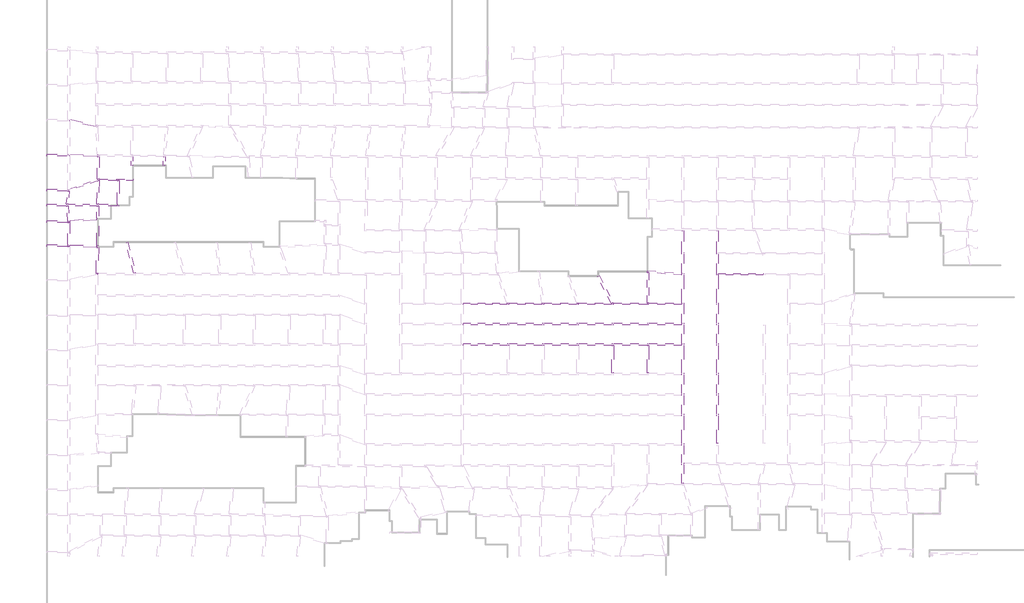
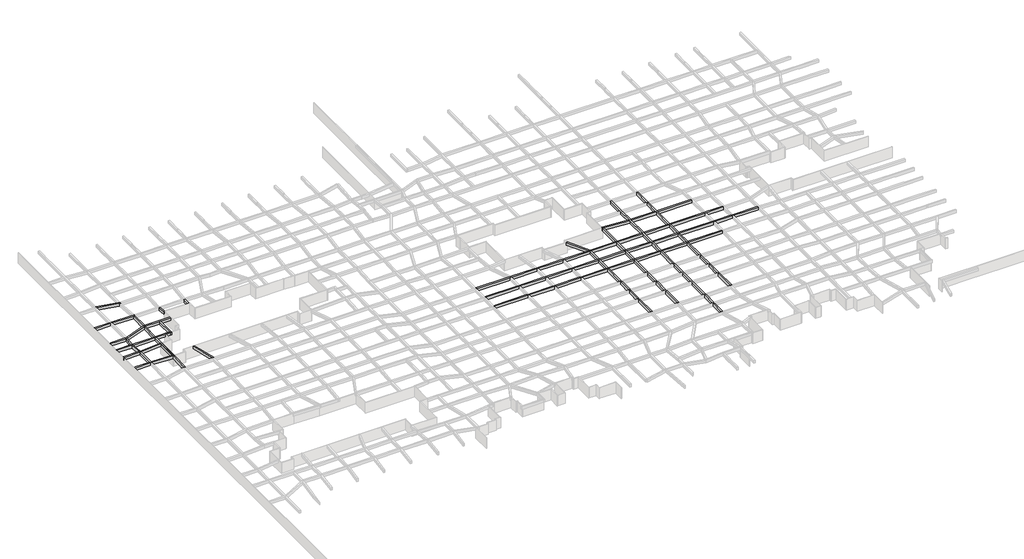
# One storey, part 34 of 45: 33 beams.
# Revit data of these elements (continued)
# Type "混凝土 - 矩形梁 : KL_beam"
#   Length [instance default] = 1524 mm
#   b = 400 mm
#   h = 800 mm
#   Structural Material [instance default] = 混凝土 - 现场浇注混凝土
#   Assembly Code = ""
# Elements 1, 2, 3, 4, 5, 6, 7, 8, 9, 10, 11, 12, 13, 14, 15, 16, 17, 18, 19, 20, 21, 22, 23, 24, 25, 26, 27, 28, 29, 30, 31, 32, 33 (IfcBeam, "混凝土 - 矩形梁 : KL_beam")
#   Comments = ""
#   Structural Material = none
#   Phase Created = 新构造
# Materials
#   "混凝土 - 现场浇注混凝土": class "混凝土", colour RGB 192 192 192, transparency 0
